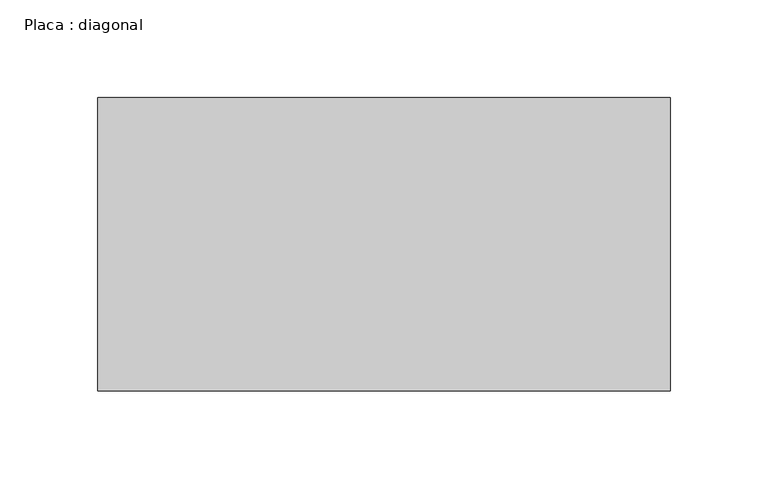
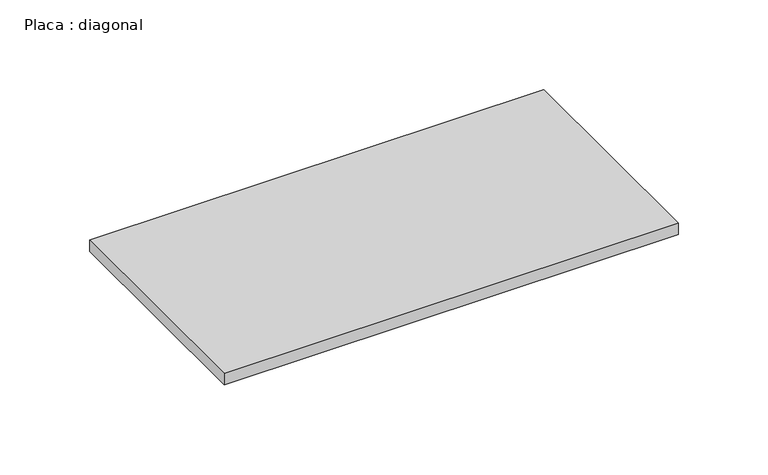
"""IFC4 building model written with IfcOpenShell, lengths in millimetres: beam geometry, Placa : diagonal."""

from ifc_helpers import new_model, si_unit, frame, origin, place, context, project, spatial, polyline, outline, extrude, source, transform, mapped, element, save


def placa_diagonal_28543f3d(model_context):
    return source(origin(), model_context, "Body", "SweptSolid", [
        extrude(outline(polyline([(146.2783525, 75.0), (146.2783525, -75.0), (-146.2783525, -75.0), (-146.2783525, 75.0), (146.2783525, 75.0)])), frame((0.0, 0.0, -4.0), z_axis=(0.0, 0.0, 1.0), x_axis=(1.0, 0.0, 0.0)), (0.0, 0.0, 1.0), 8.0),
    ])


if __name__ == "__main__":
    model = new_model("IFC4")
    model_context = context("Model", 3, world=origin())
    ifc_project = project(units=[si_unit("LENGTHUNIT", "METRE", prefix="MILLI")], contexts=[model_context])
    site = spatial("IfcSite", under=ifc_project)
    building = spatial("IfcBuilding", under=site)
    placement = place(None, origin())
    placa_diagonal_shape = placa_diagonal_28543f3d(model_context)
    element("IfcBeam", 1, ObjectType="Placa : diagonal", at=placement, inside=building, context=model_context, shape_type="MappedRepresentation", body=[
        mapped(placa_diagonal_shape, transform((0.0, 0.0, 0.0), x_axis=(1.0, 0.0, 0.0), y_axis=(0.0, 1.0, 0.0), z_axis=(0.0, 0.0, 1.0))),
    ])
    save(model, "model.ifc")

# Revit data of these elements
# Type "Placa : diagonal"
#   W = 0
#   Length [instance default] = 1.50 m
#   b = 0.15 m
#   d = 0.008 m
#   A = 0 m²
#   Structural Material [instance default] = Aço, 45-345
# Element 1 (IfcBeam, "Placa : diagonal")
#   Materials on its faces: "Aço, 45-345"
# Materials
#   "Aço, 45-345": class "Metal", colour RGB 247 247 247, transparency 0, Description = "Aço 345 MPa", Cost = 0
